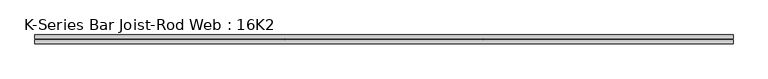
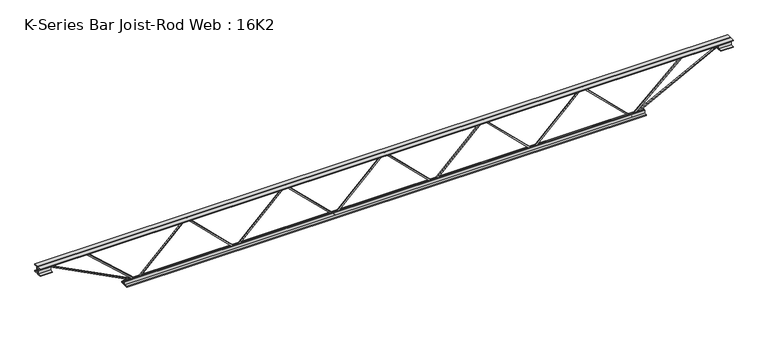
"""IFC4 building model written with IfcOpenShell, lengths in millimetres: beam geometry, K-Series Bar Joist-Rod Web : 16K2."""

from ifc_helpers import new_model, si_unit, frame, origin, place, context, project, spatial, polyline, outline, extrude, source, transform, mapped, element, save


def k_series_bar_joist_rod_web_16k2_8ccc9995(model_context):
    return source(origin(), model_context, "Body", "SweptSolid", [
        extrude(outline(polyline([(-192.0875, 406.4), (-201.6125, 406.4), (-201.6125, 411.5254109), (192.0875, 811.5754109), (192.0875, 814.0245891), (-201.6125, 1214.0745891), (-201.6125, 1219.2), (-192.0875, 1219.2), (-192.0875, 1217.9754109), (201.6125, 817.9254109), (201.6125, 807.6745891), (-192.0875, 407.6245891), (-192.0875, 406.4)])), frame((0.0, -4.7625, 0.0), z_axis=(0.0, 1.0, 0.0), x_axis=(0.0, 0.0, 1.0)), (0.0, 0.0, 1.0), 9.525),
        extrude(outline(polyline([(-192.0875, -406.4), (-201.6125, -406.4), (-201.6125, -401.2745891), (192.0875, -1.2245891), (192.0875, 1.2245891), (-201.6125, 401.2745891), (-201.6125, 406.4), (-192.0875, 406.4), (-192.0875, 405.1754109), (201.6125, 5.1254109), (201.6125, -5.1254109), (-192.0875, -405.1754109), (-192.0875, -406.4)])), frame((0.0, -4.7625, 0.0), z_axis=(0.0, 1.0, 0.0), x_axis=(0.0, 0.0, 1.0)), (0.0, 0.0, 1.0), 9.525),
        extrude(outline(polyline([(-192.0875, -1219.2), (-201.6125, -1219.2), (-201.6125, -1214.0745891), (192.0875, -814.0245891), (192.0875, -811.5754109), (-201.6125, -411.5254109), (-201.6125, -406.4), (-192.0875, -406.4), (-192.0875, -407.6245891), (201.6125, -807.6745891), (201.6125, -817.9254109), (-192.0875, -1217.9754109), (-192.0875, -1219.2)])), frame((0.0, -4.7625, 0.0), z_axis=(0.0, 1.0, 0.0), x_axis=(0.0, 0.0, 1.0)), (0.0, 0.0, 1.0), 9.525),
        extrude(outline(polyline([(-192.0875, 1219.2), (-201.6125, 1219.2), (-201.6125, 1224.3254109), (192.0875, 1624.3754109), (192.0875, 1626.8245891), (-201.6125, 2026.8745891), (-201.6125, 2032.0), (-192.0875, 2032.0), (-192.0875, 2030.7754109), (201.6125, 1630.7254109), (201.6125, 1620.4745891), (-192.0875, 1220.4245891), (-192.0875, 1219.2)])), frame((0.0, -4.7625, 0.0), z_axis=(0.0, 1.0, 0.0), x_axis=(0.0, 0.0, 1.0)), (0.0, 0.0, 1.0), 9.525),
        extrude(outline(polyline([(-192.0875, -2032.0), (-201.6125, -2032.0), (-201.6125, -2026.8745891), (192.0875, -1626.8245891), (192.0875, -1624.3754109), (-201.6125, -1224.3254109), (-201.6125, -1219.2), (-192.0875, -1219.2), (-192.0875, -1220.4245891), (201.6125, -1620.4745891), (201.6125, -1630.7254109), (-192.0875, -2030.7754109), (-192.0875, -2032.0)])), frame((0.0, -4.7625, 0.0), z_axis=(0.0, 1.0, 0.0), x_axis=(0.0, 0.0, 1.0)), (0.0, 0.0, 1.0), 9.525),
        extrude(outline(polyline([(4.7625, 203.2), (36.5125, 203.2), (36.5125, 196.85), (11.1125, 196.85), (11.1125, 171.45), (4.7625, 171.45), (4.7625, 203.2)])), frame((-2844.8, 0.0, 0.0), z_axis=(1.0, 0.0, 0.0), x_axis=(0.0, 1.0, 0.0)), (0.0, 0.0, 1.0), 5689.6),
        extrude(outline(polyline([(-4.7625, 203.2), (-4.7625, 171.45), (-11.1125, 171.45), (-11.1125, 196.85), (-36.5125, 196.85), (-36.5125, 203.2), (-4.7625, 203.2)])), frame((-2844.8, 0.0, 0.0), z_axis=(1.0, 0.0, 0.0), x_axis=(0.0, 1.0, 0.0)), (0.0, 0.0, 1.0), 5689.6),
        extrude(outline(polyline([(-4.7625, 139.7), (-36.5125, 139.7), (-36.5125, 146.05), (-11.1125, 146.05), (-11.1125, 171.45), (-4.7625, 171.45), (-4.7625, 139.7)])), frame((-2844.8, 0.0, 0.0), z_axis=(1.0, 0.0, 0.0), x_axis=(0.0, 1.0, 0.0)), (0.0, 0.0, 1.0), 101.6),
        extrude(outline(polyline([(36.5125, 139.7), (4.7625, 139.7), (4.7625, 171.45), (11.1125, 171.45), (11.1125, 146.05), (36.5125, 146.05), (36.5125, 139.7)])), frame((-2844.8, 0.0, 0.0), z_axis=(1.0, 0.0, 0.0), x_axis=(0.0, 1.0, 0.0)), (0.0, 0.0, 1.0), 101.6),
        extrude(outline(polyline([(4.7625, 139.7), (4.7625, 171.45), (11.1125, 171.45), (11.1125, 146.05), (36.5125, 146.05), (36.5125, 139.7), (4.7625, 139.7)])), frame((2743.2, 0.0, 0.0), z_axis=(1.0, 0.0, 0.0), x_axis=(0.0, 1.0, 0.0)), (0.0, 0.0, 1.0), 101.6),
        extrude(outline(polyline([(-4.7625, 139.7), (-36.5125, 139.7), (-36.5125, 146.05), (-11.1125, 146.05), (-11.1125, 171.45), (-4.7625, 171.45), (-4.7625, 139.7)])), frame((2743.2, 0.0, 0.0), z_axis=(1.0, 0.0, 0.0), x_axis=(0.0, 1.0, 0.0)), (0.0, 0.0, 1.0), 101.6),
        extrude(outline(polyline([(4.7625, -203.2), (4.7625, -171.45), (11.1125, -171.45), (11.1125, -196.85), (36.5125, -196.85), (36.5125, -203.2), (4.7625, -203.2)])), frame((-2133.6, 0.0, 0.0), z_axis=(1.0, 0.0, 0.0), x_axis=(0.0, 1.0, 0.0)), (0.0, 0.0, 1.0), 4267.2),
        extrude(outline(polyline([(-4.7625, -203.2), (-36.5125, -203.2), (-36.5125, -196.85), (-11.1125, -196.85), (-11.1125, -171.45), (-4.7625, -171.45), (-4.7625, -203.2)])), frame((-2133.6, 0.0, 0.0), z_axis=(1.0, 0.0, 0.0), x_axis=(0.0, 1.0, 0.0)), (0.0, 0.0, 1.0), 4267.2),
        extrude(outline(polyline([(0.0, -9.525), (0.0, 0.0), (800.9059433, 0.0), (800.9059433, -9.525), (0.0, -9.525)])), frame((-2745.3900559, 4.7625, 167.2209266), z_axis=(0.45985424766113764, 0.0, 0.887994409277451), x_axis=(0.887994409277451, 0.0, -0.45985424766113764)), (0.0, 0.0, 1.0), 9.525),
        extrude(outline(polyline([(0.0, -9.525), (0.0, 0.0), (548.4577012, 0.0), (548.4577012, -9.525), (0.0, -9.525)])), frame((-2441.5981113, 4.7625, 167.9210496), z_axis=(0.6715194247385565, 0.0, 0.7409869514362573), x_axis=(0.7409869514362573, 0.0, -0.6715194247385565)), (0.0, 0.0, 1.0), 9.525),
        extrude(outline(polyline([(0.0, -9.525), (0.0, 0.0), (800.9059433, 0.0), (800.9059433, -9.525), (0.0, -9.525)])), frame((2745.3900559, -4.7625, 167.2209266), z_axis=(-0.4598542476611245, 0.0, 0.8879944092774579), x_axis=(-0.8879944092774579, 0.0, -0.4598542476611245)), (0.0, 0.0, 1.0), 9.525),
        extrude(outline(polyline([(0.0, -9.525), (0.0, 0.0), (548.4577012, 0.0), (548.4577012, -9.525), (0.0, -9.525)])), frame((2441.5981113, -4.7625, 167.9210496), z_axis=(-0.6715194247385526, 0.0, 0.7409869514362606), x_axis=(-0.7409869514362606, 0.0, -0.6715194247385526)), (0.0, 0.0, 1.0), 9.525),
    ])


if __name__ == "__main__":
    model = new_model("IFC4")
    model_context = context("Model", 3, world=origin())
    ifc_project = project(units=[si_unit("LENGTHUNIT", "METRE", prefix="MILLI")], contexts=[model_context])
    site = spatial("IfcSite", under=ifc_project)
    building = spatial("IfcBuilding", under=site)
    placement = place(None, origin())
    k_series_bar_joist_rod_web_16k2_shape = k_series_bar_joist_rod_web_16k2_8ccc9995(model_context)
    element("IfcBeam", 1, ObjectType="K-Series Bar Joist-Rod Web : 16K2", at=placement, inside=building, context=model_context, shape_type="MappedRepresentation", body=[
        mapped(k_series_bar_joist_rod_web_16k2_shape, transform((0.0, 0.0, 0.0), x_axis=(1.0, 0.0, 0.0), y_axis=(0.0, 1.0, 0.0), z_axis=(0.0, 0.0, 1.0))),
    ])
    save(model, "model.ifc")

# Revit data of these elements
# Type "K-Series Bar Joist-Rod Web : 16K2"
#   Assembly Code = "B1010350"
#   Wt = 5.5
#   Web Thickness = 0' - 0 3/8"
#   Start Offset [instance default] = 0' - 0"
#   Start Extension [instance default] = 0' - 0"
#   Seat Length = 0' - 4"
#   Seat Depth = 0' - 2 1/2"
#   PanelArrayLength [instance default] = 18' - 8"
#   Panel [instance default] = 2' - 8"
#   End Offset [instance default] = 0' - 0"
#   End Extension [instance default] = 0' - 0"
#   End Panel = 2' - 8"
#   Cord Leg = 0' - 1 1/4"
#   Chord Thickness = 0' - 0 1/4"
#   Length [instance default] = 24' - 0"
#   Depth = 1' - 4"
#   PanelArrayNum [instance default] = 7
#   Structural Material = none
# Element 1 (IfcBeam, "K-Series Bar Joist-Rod Web : 16K2")
#   PanelArrayLength = 13' - 4"
#   PanelArrayNum = 5
